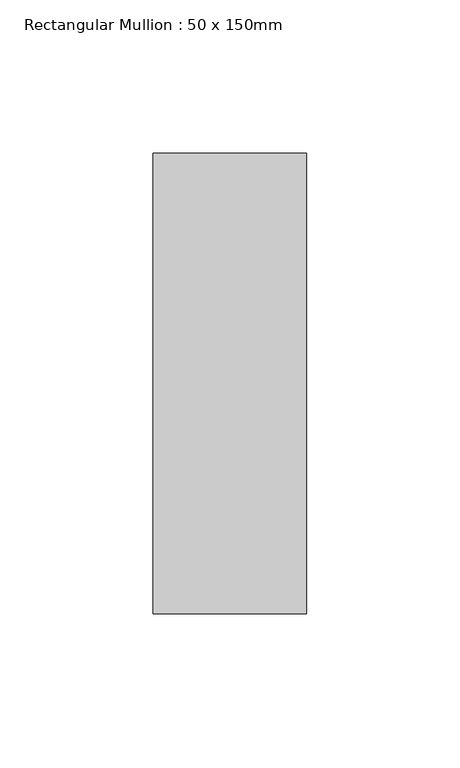
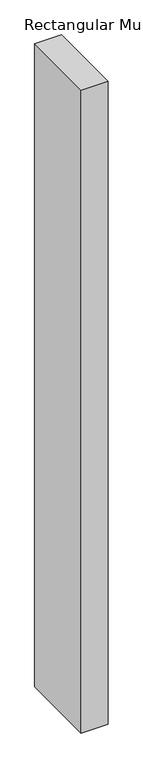
"""IFC4 building model written with IfcOpenShell, lengths in millimetres: member geometry, Rectangular Mullion : 50 x 150mm."""

from ifc_helpers import new_model, si_unit, frame, origin, place, context, project, spatial, polyline, outline, extrude, source, transform, mapped, element, save


def rectangular_mullion_50_x_150mm_ce8ae2ec(model_context):
    return source(origin(), model_context, "Body", "SweptSolid", [
        extrude(outline(polyline([(0.0, 75.0), (0.0, -75.0), (-50.0, -75.0), (-50.0, 75.0), (0.0, 75.0)])), frame((0.0, 0.0, -1266.108271), z_axis=(0.0, 0.0, 1.0), x_axis=(1.0, 0.0, 0.0)), (0.0, 0.0, 1.0), 1266.108271),
    ])


if __name__ == "__main__":
    model = new_model("IFC4")
    model_context = context("Model", 3, world=origin())
    ifc_project = project(units=[si_unit("LENGTHUNIT", "METRE", prefix="MILLI")], contexts=[model_context])
    site = spatial("IfcSite", under=ifc_project)
    building = spatial("IfcBuilding", under=site)
    placement = place(None, origin())
    rectangular_mullion_50_x_150mm_shape = rectangular_mullion_50_x_150mm_ce8ae2ec(model_context)
    element("IfcMember", 1, ObjectType="Rectangular Mullion : 50 x 150mm", at=placement, inside=building, context=model_context, shape_type="MappedRepresentation", body=[
        mapped(rectangular_mullion_50_x_150mm_shape, transform((0.0, 0.0, 0.0), x_axis=(1.0, 0.0, 0.0), y_axis=(0.0, 1.0, 0.0), z_axis=(0.0, 0.0, 1.0))),
    ])
    save(model, "model.ifc")

# Revit data of these elements
# Type "Rectangular Mullion : 50 x 150mm"
#   built-in parameter 1007304 = 0.492126 (stored number, unit not read)
#   built-in parameter 1007301 = 0.082021 (stored number, unit not read)
#   built-in parameter 1007300 = 0.082021 (stored number, unit not read)
# Element 1 (IfcMember, "Rectangular Mullion : 50 x 150mm")
#   Materials on its faces: "Aluminium"
# Materials
#   "Aluminium": class "Metal", colour RGB 247 247 247, transparency 0, Description = "Aluminium 6061", Cost = 0
